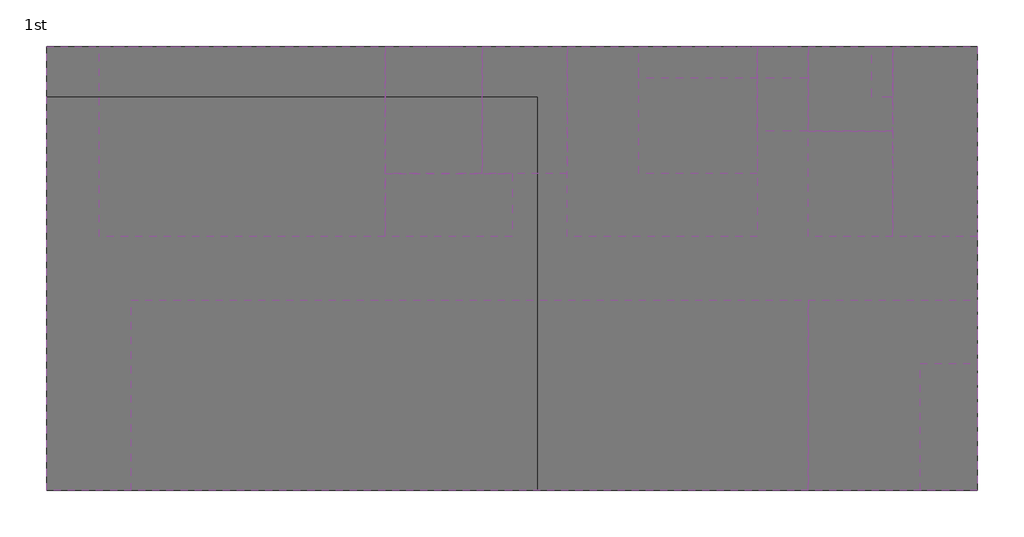
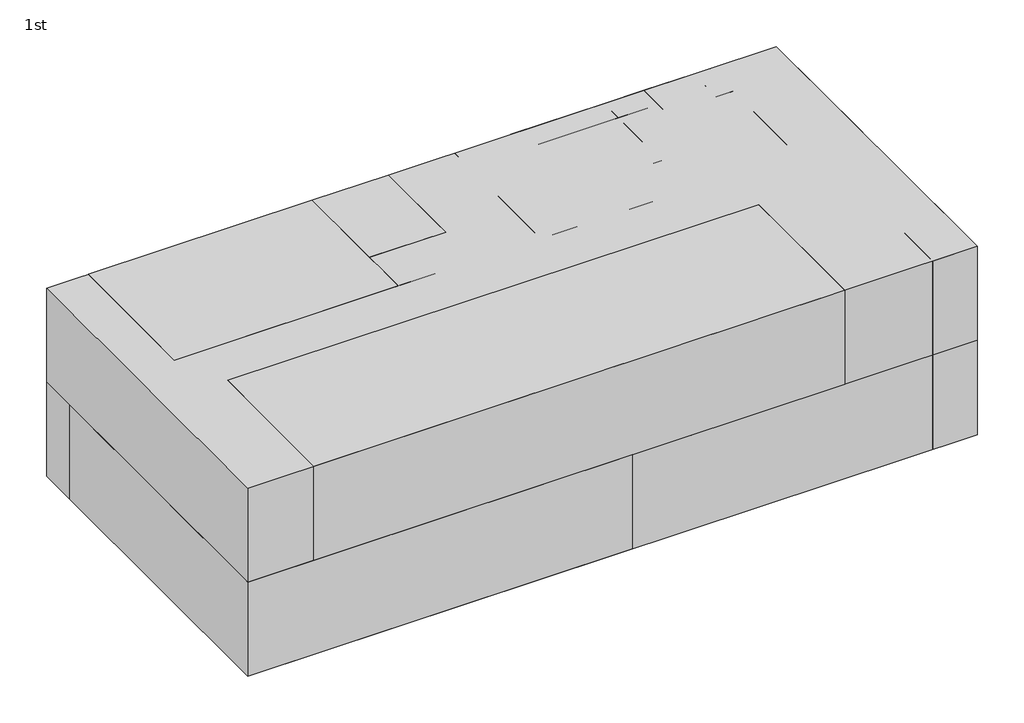
# One storey: 23 proxies.
"""IFC4 building model written with IfcOpenShell, lengths in millimetres."""

import ifcopenshell
import ifcopenshell.guid

model = None  # the IFC model being written
_history = None  # IfcOwnerHistory: only IFC2X3 demands one
_inside = {}  # id of a spatial element -> (the spatial element, [elements in it])
_under = {}  # id of a project, library or spatial element -> (it, [spatial elements below it])
_declared = {}  # id of a project -> (the project, [libraries it declares])
_typed = {}  # id of a type object -> (the type object, [elements of that type])
_made_of = {}  # id of a material, layer set ... -> (it, [elements and type objects made of it])


def new_model(schema):
    """Start an empty IFC model of exactly this schema.

    Asked for "IFC4X3", IfcOpenShell would pick the latest addendum, in which some entities
    have other attributes; the version numbers below select the first issue.
    IFC2X3 requires an IfcOwnerHistory on every rooted entity: one is made here for all.
    """
    global model, _history
    if schema == "IFC4X3":
        model = ifcopenshell.file(schema_version=(4, 3, 0, 0))
    else:
        model = ifcopenshell.file(schema=schema)
    _inside.clear()
    _under.clear()
    _declared.clear()
    _typed.clear()
    _made_of.clear()
    _history = None
    if model.schema == "IFC2X3":
        org = make("IfcOrganization", Name="unknown")
        user = make(
            "IfcPersonAndOrganization",
            ThePerson=make("IfcPerson", FamilyName="unknown"),
            TheOrganization=org,
        )
        app = make(
            "IfcApplication",
            ApplicationDeveloper=org,
            Version="unknown",
            ApplicationFullName="unknown",
            ApplicationIdentifier="unknown",
        )
        _history = make(
            "IfcOwnerHistory",
            OwningUser=user,
            OwningApplication=app,
            ChangeAction="ADDED",
            CreationDate=0,
        )
    return model


def make(cls, **values):
    """One entity of the class cls with the attributes given. An attribute that is None is left unset."""
    return model.create_entity(
        cls, **{name: value for name, value in values.items() if value is not None}
    )


def rooted(cls, **values):
    """An entity with a GlobalId (a new one), such as an element, a storey or a relation."""
    return make(cls, GlobalId=ifcopenshell.guid.new(), OwnerHistory=_history, **values)


def si_unit(unit_type, name, prefix=None):
    """IfcSIUnit, for example si_unit("LENGTHUNIT", "METRE", prefix="MILLI")."""
    return make("IfcSIUnit", UnitType=unit_type, Prefix=prefix, Name=name)


def assignment(units):
    """IfcUnitAssignment: the units of a project."""
    return None if units is None else make("IfcUnitAssignment", Units=units)


def point(xyz):
    """IfcCartesianPoint."""
    return None if xyz is None else make("IfcCartesianPoint", Coordinates=xyz)


def direction(xyz):
    """IfcDirection."""
    return None if xyz is None else make("IfcDirection", DirectionRatios=xyz)


def frame(location, z_axis=None, x_axis=None):
    """IfcAxis2Placement3D, a coordinate frame: its origin and axes. An axis left out is left unset."""
    return make(
        "IfcAxis2Placement3D",
        Location=point(location),
        Axis=direction(z_axis),
        RefDirection=direction(x_axis),
    )


def origin():
    """The frame at (0, 0, 0) with its axes left unset."""
    return frame((0.0, 0.0, 0.0))


def origin_with_axes():
    """The frame at (0, 0, 0) with the z axis (0, 0, 1) and the x axis (1, 0, 0) written out."""
    return frame((0.0, 0.0, 0.0), z_axis=(0.0, 0.0, 1.0), x_axis=(1.0, 0.0, 0.0))


def place(relative_to, where):
    """IfcLocalPlacement: puts the frame where relative to a parent placement (None: the world)."""
    return make(
        "IfcLocalPlacement", PlacementRelTo=relative_to, RelativePlacement=where
    )


def context(
    kind, dimensions, precision=None, world=None, true_north=None, identifier=None
):
    """IfcGeometricRepresentationContext, for example the 3D "Model" context."""
    return make(
        "IfcGeometricRepresentationContext",
        ContextIdentifier=identifier,
        ContextType=kind,
        CoordinateSpaceDimension=dimensions,
        Precision=precision,
        WorldCoordinateSystem=world,
        TrueNorth=true_north,
    )


def project(units=None, contexts=None):
    """IfcProject with its units and contexts."""
    return rooted(
        "IfcProject",
        Name="project",
        RepresentationContexts=contexts,
        UnitsInContext=assignment(units),
    )


def spatial(cls, under=None, at=None, **own):
    """A site, building, storey or space (cls), placed at a placement, below another one or the project."""
    s = rooted(cls, ObjectPlacement=at, **own)
    if under is not None:
        _under.setdefault(under.id(), (under, []))[1].append(s)
    return s


def polyline(points):
    """IfcPolyline through the points."""
    return make("IfcPolyline", Points=[point(p) for p in points])


def outline(outer, holes=None, kind="AREA"):
    """IfcArbitraryClosedProfileDef: a profile drawn as a closed curve; with holes, ...WithVoids."""
    if holes is None:
        return make("IfcArbitraryClosedProfileDef", ProfileType=kind, OuterCurve=outer)
    return make(
        "IfcArbitraryProfileDefWithVoids",
        ProfileType=kind,
        OuterCurve=outer,
        InnerCurves=holes,
    )


def extrude(swept, where, along, depth):
    """IfcExtrudedAreaSolid: the profile swept, set in the frame where, extruded along a direction by depth."""
    return make(
        "IfcExtrudedAreaSolid",
        SweptArea=swept,
        Position=where,
        ExtrudedDirection=direction(along),
        Depth=depth,
    )


def shape(context_of_items, identifier, shape_type, items):
    """IfcShapeRepresentation: the items that make up one representation, for example the "Body"."""
    return make(
        "IfcShapeRepresentation",
        ContextOfItems=context_of_items,
        RepresentationIdentifier=identifier,
        RepresentationType=shape_type,
        Items=items,
    )


def source(mapping_origin, context_of_items, identifier, shape_type, items):
    """IfcRepresentationMap: a shape defined once, which mapped items show again and again."""
    return make(
        "IfcRepresentationMap",
        MappingOrigin=mapping_origin,
        MappedRepresentation=shape(context_of_items, identifier, shape_type, items),
    )


def transform(
    local_origin,
    x_axis=None,
    y_axis=None,
    z_axis=None,
    scale=None,
    scale2=None,
    scale3=None,
    uniform=True,
):
    """IfcCartesianTransformationOperator3D, or its non-uniform kind. x_axis, y_axis, z_axis: its Axis1, 2, 3."""
    if uniform:
        return make(
            "IfcCartesianTransformationOperator3D",
            Axis1=direction(x_axis),
            Axis2=direction(y_axis),
            LocalOrigin=point(local_origin),
            Scale=scale,
            Axis3=direction(z_axis),
        )
    return make(
        "IfcCartesianTransformationOperator3DnonUniform",
        Axis1=direction(x_axis),
        Axis2=direction(y_axis),
        LocalOrigin=point(local_origin),
        Scale=scale,
        Axis3=direction(z_axis),
        Scale2=scale2,
        Scale3=scale3,
    )


def mapped(mapping_source, mapping_target):
    """IfcMappedItem: shows the shape of a source again, moved by a transform."""
    return make(
        "IfcMappedItem", MappingSource=mapping_source, MappingTarget=mapping_target
    )


def made_of(thing, what):
    """Note that an element or type object is made of a material, layer set ...; save() writes the relation."""
    if what is not None:
        _made_of.setdefault(what.id(), (what, []))[1].append(thing)
    return thing


def element(
    cls,
    number,
    at=None,
    inside=None,
    cuts=None,
    type_object=None,
    material=None,
    context=None,
    identifier="Body",
    shape_type=None,
    held_by="IfcProductDefinitionShape",
    body=None,
    shapes=None,
    **own,
):
    """One element of the class cls, such as IfcWall. Its Tag is "e" and its number.

    at: its placement. inside: the storey or other place that contains it. cuts: it is an
    opening in that element (IfcRelVoidsElement). A single representation is given by context,
    identifier, shape_type and body (its items); several are given by shapes. held_by: the class
    of the entity that holds the representations. save() writes the other relations.
    """
    e = rooted(cls, Tag="e%d" % number, ObjectPlacement=at, **own)
    if body is not None:
        shapes = [shape(context, identifier, shape_type, body)]
    if shapes is not None:
        e.Representation = make(held_by, Representations=shapes)
    if inside is not None:
        _inside.setdefault(inside.id(), (inside, []))[1].append(e)
    if cuts is not None:
        rooted(
            "IfcRelVoidsElement", RelatingBuildingElement=cuts, RelatedOpeningElement=e
        )
    if type_object is not None:
        _typed.setdefault(type_object.id(), (type_object, []))[1].append(e)
    return made_of(e, material)


def aggregate(whole, parts):
    """IfcRelAggregates: a whole, such as a stair, and the parts it consists of."""
    return rooted("IfcRelAggregates", RelatingObject=whole, RelatedObjects=parts)


def save(model, path):
    """Write the relations noted so far, then the file.

    IfcRelAggregates (storeys below a building ...), IfcRelContainedInSpatialStructure (elements
    in a storey), IfcRelDefinesByType, IfcRelAssociatesMaterial and IfcRelDeclares: one each for
    every whole, place, type object, material and project.
    """
    for whole, parts in _under.values():
        aggregate(whole, parts)
    for where, things in _inside.values():
        rooted(
            "IfcRelContainedInSpatialStructure",
            RelatedElements=things,
            RelatingStructure=where,
        )
    for kind, things in _typed.values():
        rooted("IfcRelDefinesByType", RelatedObjects=things, RelatingType=kind)
    for what, things in _made_of.values():
        rooted("IfcRelAssociatesMaterial", RelatedObjects=things, RelatingMaterial=what)
    for by, libraries in _declared.values():
        rooted("IfcRelDeclares", RelatingContext=by, RelatedDefinitions=libraries)
    model.write(path)


def generic_models_29bcd6f9(model_context):
    return source(origin(), model_context, "Body", "SweptSolid", [
        extrude(outline(polyline([(2000.0, 4500.0), (2000.0, -4500.0), (-2000.0, -4500.0), (-2000.0, 4500.0), (2000.0, 4500.0)])), origin_with_axes(), (0.0, 0.0, 1.0), 6000.0),
    ])


def generic_models_d82b1902(model_context):
    return source(origin(), model_context, "Body", "SweptSolid", [
        extrude(outline(polyline([(9300.0, 11600.0), (9300.0, -11600.0), (-9300.0, -11600.0), (-9300.0, 11600.0), (9300.0, 11600.0)])), origin_with_axes(), (0.0, 0.0, 1.0), 6000.0),
    ])


def generic_models_5634f436(model_context):
    return source(origin(), model_context, "Body", "SweptSolid", [
        extrude(outline(polyline([(1350.0, 3000.0), (1350.0, -3000.0), (-1350.0, -3000.0), (-1350.0, 3000.0), (1350.0, 3000.0)])), origin_with_axes(), (0.0, 0.0, 1.0), 6000.0),
    ])


def generic_models_57c7875f(model_context):
    return source(origin(), model_context, "Body", "SweptSolid", [
        extrude(outline(polyline([(4500.0, 16000.0), (4500.0, -16000.0), (-4500.0, -16000.0), (-4500.0, 16000.0), (4500.0, 16000.0)])), origin_with_axes(), (0.0, 0.0, 1.0), 6000.0),
    ])


def generic_models_7bff30ad(model_context):
    return source(origin(), model_context, "Body", "SweptSolid", [
        extrude(outline(polyline([(2000.0, 2000.0), (2000.0, -2000.0), (-2000.0, -2000.0), (-2000.0, 2000.0), (2000.0, 2000.0)])), origin_with_axes(), (0.0, 0.0, 1.0), 6000.0),
    ])


def generic_models_5b7b272c(model_context):
    return source(origin(), model_context, "Body", "SweptSolid", [
        extrude(outline(polyline([(2000.0, 2500.0), (2000.0, -2500.0), (-2000.0, -2500.0), (-2000.0, 2500.0), (2000.0, 2500.0)])), origin_with_axes(), (0.0, 0.0, 1.0), 6000.0),
    ])


def generic_models_47b98be1(model_context):
    return source(origin(), model_context, "Body", "SweptSolid", [
        extrude(outline(polyline([(1200.0, 2000.0), (1200.0, -2000.0), (-1200.0, -2000.0), (-1200.0, 2000.0), (1200.0, 2000.0)])), origin_with_axes(), (0.0, 0.0, 1.0), 6000.0),
    ])


def generic_models_7a053eeb(model_context):
    return source(origin(), model_context, "Body", "SweptSolid", [
        extrude(outline(polyline([(1200.0, 750.0), (1200.0, -750.0), (-1200.0, -750.0), (-1200.0, 750.0), (1200.0, 750.0)])), origin_with_axes(), (0.0, 0.0, 1.0), 6000.0),
    ])


def generic_models_ec17d728(model_context):
    return source(origin(), model_context, "Body", "SweptSolid", [
        extrude(outline(polyline([(2800.0, 3000.0), (2800.0, -3000.0), (-2800.0, -3000.0), (-2800.0, 3000.0), (2800.0, 3000.0)])), origin_with_axes(), (0.0, 0.0, 1.0), 6000.0),
    ])


def generic_models_85897e09(model_context):
    return source(origin(), model_context, "Body", "SweptSolid", [
        extrude(outline(polyline([(2800.0, 750.0), (2800.0, -750.0), (-2800.0, -750.0), (-2800.0, 750.0), (2800.0, 750.0)])), origin_with_axes(), (0.0, 0.0, 1.0), 6000.0),
    ])


def generic_models_b79df083(model_context):
    return source(origin(), model_context, "Body", "SweptSolid", [
        extrude(outline(polyline([(4500.0, 4500.0), (4500.0, -4500.0), (-4500.0, -4500.0), (-4500.0, 4500.0), (4500.0, 4500.0)])), origin_with_axes(), (0.0, 0.0, 1.0), 6000.0),
    ])


def generic_models_98b71764(model_context):
    return source(origin(), model_context, "Body", "SweptSolid", [
        extrude(outline(polyline([(2000.0, 3000.0), (2000.0, -3000.0), (-2000.0, -3000.0), (-2000.0, 3000.0), (2000.0, 3000.0)])), origin_with_axes(), (0.0, 0.0, 1.0), 6000.0),
    ])


def generic_models_1a87c0f4(model_context):
    return source(origin(), model_context, "Body", "SweptSolid", [
        extrude(outline(polyline([(2300.0, 3000.0), (2300.0, -3000.0), (-2300.0, -3000.0), (-2300.0, 3000.0), (2300.0, 3000.0)])), origin_with_axes(), (0.0, 0.0, 1.0), 6000.0),
    ])


def generic_models_df3bc381(model_context):
    return source(origin(), model_context, "Body", "SweptSolid", [
        extrude(outline(polyline([(4500.0, 6750.0), (4500.0, -6750.0), (-4500.0, -6750.0), (-4500.0, 6750.0), (4500.0, 6750.0)])), origin_with_axes(), (0.0, 0.0, 1.0), 6000.0),
    ])


def generic_models_542cc789(model_context):
    return source(origin(), model_context, "Body", "SweptSolid", [
        extrude(outline(polyline([(1500.0, 3000.0), (1500.0, -3000.0), (-1500.0, -3000.0), (-1500.0, 3000.0), (1500.0, 3000.0)])), origin_with_axes(), (0.0, 0.0, 1.0), 6000.0),
    ])


def generic_models_4d084078(model_context):
    return source(origin(), model_context, "Body", "SweptSolid", [
        extrude(outline(polyline([(4000.0, 4500.0), (4000.0, -4500.0), (-4000.0, -4500.0), (-4000.0, 4500.0), (4000.0, 4500.0)])), origin_with_axes(), (0.0, 0.0, 1.0), 6000.0),
    ])


def generic_models_7e8091d6(model_context):
    return source(origin(), model_context, "Body", "SweptSolid", [
        extrude(outline(polyline([(22000.0, 10500.0), (22000.0, -10500.0), (-22000.0, -10500.0), (-22000.0, 10500.0), (22000.0, 10500.0)])), origin_with_axes(), (0.0, 0.0, 1.0), 6000.0),
    ])


def generic_models_b146db3b(model_context):
    return source(origin(), model_context, "Body", "SweptSolid", [
        extrude(outline(polyline([(10500.0, 22000.0), (10500.0, -22000.0), (-10500.0, -22000.0), (-10500.0, 22000.0), (10500.0, 22000.0)])), origin_with_axes(), (0.0, 0.0, 1.0), 6000.0),
    ])


def generic_models_21888712(model_context):
    return source(origin(), model_context, "Body", "SweptSolid", [
        extrude(outline(polyline([(500.0, 1200.0), (500.0, -1200.0), (-500.0, -1200.0), (-500.0, 1200.0), (500.0, 1200.0)])), origin_with_axes(), (0.0, 0.0, 1.0), 6000.0),
    ])


model = new_model("IFC4")

# Units and contexts
model_context = context("Model", 3, world=origin())
ifc_project = project(units=[si_unit("LENGTHUNIT", "METRE", prefix="MILLI")], contexts=[model_context])

# Site, building, storey
site = spatial("IfcSite", under=ifc_project)
building = spatial("IfcBuilding", under=site)
storey = spatial("IfcBuildingStorey", under=building, Name="1st", Elevation=6000.0)

# Proxies
placement = place(None, origin())
element("IfcBuildingElementProxy", 1, Name="Space Planning Box_hec : Space Planning Box_hec", ObjectType="Space Planning Box_hec : Space Planning Box_hec", at=placement, inside=storey, context=model_context, shape_type="SweptSolid", body=[
    extrude(outline(polyline([(89459.6521483, 163923.8614395), (68659.6521483, 163923.8614395), (68659.6521483, 182523.8614395), (85459.6521483, 182523.8614395), (85459.6521483, 175923.8614395), (89459.6521483, 175923.8614395), (89459.6521483, 163923.8614395)])), frame((0.0, 0.0, 6000.0), z_axis=(0.0, 0.0, 1.0), x_axis=(1.0, 0.0, 0.0)), (0.0, 0.0, 1.0), 6000.0),
])
element("IfcBuildingElementProxy", 2, Name="Space Planning Box_hec : Space Planning Box_hec", ObjectType="Space Planning Box_hec : Space Planning Box_hec", at=placement, inside=storey, context=model_context, shape_type="SweptSolid", body=[
    extrude(outline(polyline([(89459.6521483, 184923.8614395), (89459.6521483, 175923.8614395), (85459.6521483, 175923.8614395), (85459.6521483, 184923.8614395), (89459.6521483, 184923.8614395)])), frame((0.0, 0.0, 6000.0), z_axis=(0.0, 0.0, 1.0), x_axis=(1.0, 0.0, 0.0)), (0.0, 0.0, 1.0), 6000.0),
])
generic_models_shape = generic_models_29bcd6f9(model_context)
element("IfcBuildingElementProxy", 3, Name="Space Planning Box_hec : Space Planning Box_hec", ObjectType="Space Planning Box_hec : Space Planning Box_hec", at=placement, inside=storey, context=model_context, shape_type="MappedRepresentation", body=[
    mapped(generic_models_shape, transform((87459.6521483, 180423.8614395, 12000.0), x_axis=(1.0, 0.0, 0.0), y_axis=(0.0, 1.0, 0.0), z_axis=(0.0, 0.0, 1.0))),
])
generic_models_2_shape = generic_models_d82b1902(model_context)
element("IfcBuildingElementProxy", 4, Name="Space Planning Box_hec : Space Planning Box_hec", ObjectType="Space Planning Box_hec : Space Planning Box_hec", at=placement, inside=storey, context=model_context, shape_type="MappedRepresentation", body=[
    mapped(generic_models_2_shape, transform((57059.6521483, 173223.8614395, 6000.0), x_axis=(0.0, -1.0, 0.0), y_axis=(1.0, 0.0, 0.0), z_axis=(0.0, 0.0, 1.0))),
])
generic_models_3_shape = generic_models_5634f436(model_context)
element("IfcBuildingElementProxy", 5, Name="Space Planning Box_hec : Space Planning Box_hec", ObjectType="Space Planning Box_hec : Space Planning Box_hec", at=placement, inside=storey, context=model_context, shape_type="MappedRepresentation", body=[
    mapped(generic_models_3_shape, transform((88109.6521483, 166923.8614395, 6000.0), x_axis=(1.0, 0.0, 0.0), y_axis=(0.0, 1.0, 0.0), z_axis=(0.0, 0.0, 1.0))),
])
element("IfcBuildingElementProxy", 6, Name="Space Planning Box_hec : Space Planning Box_hec", ObjectType="Space Planning Box_hec : Space Planning Box_hec", at=placement, inside=storey, context=model_context, shape_type="MappedRepresentation", body=[
    mapped(generic_models_3_shape, transform((88109.6521483, 166923.8614395, 12000.0), x_axis=(1.0, 0.0, 0.0), y_axis=(0.0, 1.0, 0.0), z_axis=(0.0, 0.0, 1.0))),
])
generic_models_4_shape = generic_models_57c7875f(model_context)
element("IfcBuildingElementProxy", 7, Name="Space Planning Box_hec : Space Planning Box_hec", ObjectType="Space Planning Box_hec : Space Planning Box_hec", at=placement, inside=storey, context=model_context, shape_type="MappedRepresentation", body=[
    mapped(generic_models_4_shape, transform((65459.6521483, 168423.8614395, 12000.0), x_axis=(0.0, -1.0, 0.0), y_axis=(1.0, 0.0, 0.0), z_axis=(0.0, 0.0, 1.0))),
])
generic_models_5_shape = generic_models_7bff30ad(model_context)
element("IfcBuildingElementProxy", 8, Name="Space Planning Box_hec : Space Planning Box_hec", ObjectType="Space Planning Box_hec : Space Planning Box_hec", at=placement, inside=storey, context=model_context, shape_type="MappedRepresentation", body=[
    mapped(generic_models_5_shape, transform((83459.6521483, 182923.8614395, 12000.0), x_axis=(1.0, 0.0, 0.0), y_axis=(0.0, 1.0, 0.0), z_axis=(0.0, 0.0, 1.0))),
])
generic_models_6_shape = generic_models_5b7b272c(model_context)
element("IfcBuildingElementProxy", 9, Name="Space Planning Box_hec : Space Planning Box_hec", ObjectType="Space Planning Box_hec : Space Planning Box_hec", at=placement, inside=storey, context=model_context, shape_type="MappedRepresentation", body=[
    mapped(generic_models_6_shape, transform((83459.6521483, 178423.8614395, 12000.0), x_axis=(1.0, 0.0, 0.0), y_axis=(0.0, 1.0, 0.0), z_axis=(0.0, 0.0, 1.0))),
])
generic_models_7_shape = generic_models_47b98be1(model_context)
element("IfcBuildingElementProxy", 10, Name="Space Planning Box_hec : Space Planning Box_hec", ObjectType="Space Planning Box_hec : Space Planning Box_hec", at=placement, inside=storey, context=model_context, shape_type="MappedRepresentation", body=[
    mapped(generic_models_7_shape, transform((80259.6521483, 182923.8614395, 12000.0), x_axis=(1.0, 0.0, 0.0), y_axis=(0.0, 1.0, 0.0), z_axis=(0.0, 0.0, 1.0))),
])
generic_models_8_shape = generic_models_7a053eeb(model_context)
element("IfcBuildingElementProxy", 11, Name="Space Planning Box_hec : Space Planning Box_hec", ObjectType="Space Planning Box_hec : Space Planning Box_hec", at=placement, inside=storey, context=model_context, shape_type="MappedRepresentation", body=[
    mapped(generic_models_8_shape, transform((80259.6521483, 184173.8614395, 12000.0), x_axis=(1.0, 0.0, 0.0), y_axis=(0.0, 1.0, 0.0), z_axis=(0.0, 0.0, 1.0))),
])
generic_models_9_shape = generic_models_ec17d728(model_context)
element("IfcBuildingElementProxy", 12, Name="Space Planning Box_hec : Space Planning Box_hec", ObjectType="Space Planning Box_hec : Space Planning Box_hec", at=placement, inside=storey, context=model_context, shape_type="MappedRepresentation", body=[
    mapped(generic_models_9_shape, transform((76259.6521483, 181923.8614395, 12000.0), x_axis=(1.0, 0.0, 0.0), y_axis=(0.0, 1.0, 0.0), z_axis=(0.0, 0.0, 1.0))),
])
generic_models_10_shape = generic_models_85897e09(model_context)
element("IfcBuildingElementProxy", 13, Name="Space Planning Box_hec : Space Planning Box_hec", ObjectType="Space Planning Box_hec : Space Planning Box_hec", at=placement, inside=storey, context=model_context, shape_type="MappedRepresentation", body=[
    mapped(generic_models_10_shape, transform((76259.6521483, 184173.8614395, 12000.0), x_axis=(1.0, 0.0, 0.0), y_axis=(0.0, 1.0, 0.0), z_axis=(0.0, 0.0, 1.0))),
])
generic_models_11_shape = generic_models_b79df083(model_context)
element("IfcBuildingElementProxy", 14, Name="Space Planning Box_hec : Space Planning Box_hec", ObjectType="Space Planning Box_hec : Space Planning Box_hec", at=placement, inside=storey, context=model_context, shape_type="MappedRepresentation", body=[
    mapped(generic_models_11_shape, transform((74559.6521483, 180423.8614395, 12000.0), x_axis=(1.0, 0.0, 0.0), y_axis=(0.0, 1.0, 0.0), z_axis=(0.0, 0.0, 1.0))),
])
generic_models_12_shape = generic_models_98b71764(model_context)
element("IfcBuildingElementProxy", 15, Name="Space Planning Box_hec : Space Planning Box_hec", ObjectType="Space Planning Box_hec : Space Planning Box_hec", at=placement, inside=storey, context=model_context, shape_type="MappedRepresentation", body=[
    mapped(generic_models_12_shape, transform((68059.6521483, 181923.8614395, 12000.0), x_axis=(1.0, 0.0, 0.0), y_axis=(0.0, 1.0, 0.0), z_axis=(0.0, 0.0, 1.0))),
])
generic_models_13_shape = generic_models_1a87c0f4(model_context)
element("IfcBuildingElementProxy", 16, Name="Space Planning Box_hec : Space Planning Box_hec", ObjectType="Space Planning Box_hec : Space Planning Box_hec", at=placement, inside=storey, context=model_context, shape_type="MappedRepresentation", body=[
    mapped(generic_models_13_shape, transform((63759.6521483, 181923.8614395, 12000.0), x_axis=(1.0, 0.0, 0.0), y_axis=(0.0, 1.0, 0.0), z_axis=(0.0, 0.0, 1.0))),
])
generic_models_14_shape = generic_models_df3bc381(model_context)
element("IfcBuildingElementProxy", 17, Name="Space Planning Box_hec : Space Planning Box_hec", ObjectType="Space Planning Box_hec : Space Planning Box_hec", at=placement, inside=storey, context=model_context, shape_type="MappedRepresentation", body=[
    mapped(generic_models_14_shape, transform((54709.6521483, 180423.8614395, 12000.0), x_axis=(0.0, -1.0, 0.0), y_axis=(1.0, 0.0, 0.0), z_axis=(0.0, 0.0, 1.0))),
])
generic_models_15_shape = generic_models_542cc789(model_context)
element("IfcBuildingElementProxy", 18, Name="Space Planning Box_hec : Space Planning Box_hec", ObjectType="Space Planning Box_hec : Space Planning Box_hec", at=placement, inside=storey, context=model_context, shape_type="MappedRepresentation", body=[
    mapped(generic_models_15_shape, transform((64459.6521483, 177423.8614395, 12000.0), x_axis=(0.0, -1.0, 0.0), y_axis=(1.0, 0.0, 0.0), z_axis=(0.0, 0.0, 1.0))),
])
generic_models_16_shape = generic_models_4d084078(model_context)
element("IfcBuildingElementProxy", 19, Name="Space Planning Box_hec : Space Planning Box_hec", ObjectType="Space Planning Box_hec : Space Planning Box_hec", at=placement, inside=storey, context=model_context, shape_type="MappedRepresentation", body=[
    mapped(generic_models_16_shape, transform((85459.6521483, 168423.8614395, 12000.0), x_axis=(1.0, 0.0, 0.0), y_axis=(0.0, 1.0, 0.0), z_axis=(0.0, 0.0, 1.0))),
])
generic_models_17_shape = generic_models_7e8091d6(model_context)
element("IfcBuildingElementProxy", 20, Name="Space Planning Box_hec : Space Planning Box_hec", ObjectType="Space Planning Box_hec : Space Planning Box_hec", at=placement, inside=storey, context=model_context, shape_type="MappedRepresentation", body=[
    mapped(generic_models_17_shape, transform((67459.6521483, 174423.8614395, 12000.0), x_axis=(1.0, 0.0, 0.0), y_axis=(0.0, 1.0, 0.0), z_axis=(0.0, 0.0, 1.0))),
])
generic_models_18_shape = generic_models_b146db3b(model_context)
element("IfcBuildingElementProxy", 21, Name="Space Planning Box_hec : Space Planning Box_hec", ObjectType="Space Planning Box_hec : Space Planning Box_hec", at=placement, inside=storey, context=model_context, shape_type="MappedRepresentation", body=[
    mapped(generic_models_18_shape, transform((67459.6521483, 174423.8614395, 6000.0), x_axis=(0.0, -1.0, 0.0), y_axis=(1.0, 0.0, 0.0), z_axis=(0.0, 0.0, 1.0))),
])
generic_models_19_shape = generic_models_21888712(model_context)
element("IfcBuildingElementProxy", 22, Name="Space Planning Box_hec : Space Planning Box_hec", ObjectType="Space Planning Box_hec : Space Planning Box_hec", at=placement, inside=storey, context=model_context, shape_type="MappedRepresentation", body=[
    mapped(generic_models_19_shape, transform((84959.6521483, 183723.8614395, 6000.0), x_axis=(1.0, 0.0, 0.0), y_axis=(0.0, 1.0, 0.0), z_axis=(0.0, 0.0, 1.0))),
])
element("IfcBuildingElementProxy", 23, Name="Space Planning Box_hec : Space Planning Box_hec", ObjectType="Space Planning Box_hec : Space Planning Box_hec", at=placement, inside=storey, context=model_context, shape_type="MappedRepresentation", body=[
    mapped(generic_models_19_shape, transform((84959.6521483, 183723.8614395, 12000.0), x_axis=(1.0, 0.0, 0.0), y_axis=(0.0, 1.0, 0.0), z_axis=(0.0, 0.0, 1.0))),
])

save(model, "model.ifc")

# Revit data of these elements
# Type "Space Planning Box_hec : Space Planning Box_hec"
#   Type Comments = "..."
#   Room Name [instance default] = "?"
#   Interior Finish [instance default] = ""
#   Exterior Finish [instance default] = ""
#   Department [instance default] = ""
#   Assembly Code = "..."
#   Width [instance default] = 1524 mm
#   Program Area [instance default] = 0.00 m²
#   Length [instance default] = 1524 mm
#   Height [instance default] = 1524 mm
#   Area [instance default] = 2.32258 m²
#   Fill Color [instance default] = Cyan
#   Default Elevation = 0
# Element 1 (IfcBuildingElementProxy, "Space Planning Box_hec : Space Planning Box_hec")
#   Room Name = "Electrical Room"
#   Interior Finish = "IF1"
#   Exterior Finish = "EF1"
#   Department = "EL"
#   Width = 18600 mm
#   Program Area = 238.08 m²
#   Length = 20800 mm
#   Height = 6000 mm
#   Area = 386.88 m²
#   Fill Color = Blue
#   Phase Created = New Construction
#   Materials on its faces: "Blue"
# Element 2 (IfcBuildingElementProxy, "Space Planning Box_hec : Space Planning Box_hec")
#   Room Name = "Stairway"
#   Interior Finish = "IF2"
#   Exterior Finish = "EF1"
#   Department = "AR"
#   Width = 4000 mm
#   Program Area = 36.00 m²
#   Length = 9000 mm
#   Height = 6000 mm
#   Area = 36.00 m²
#   Fill Color = Lavender
#   Phase Created = New Construction
#   Materials on its faces: "Lavender"
# Element 3 (IfcBuildingElementProxy, "Space Planning Box_hec : Space Planning Box_hec")
#   Room Name = "Stairway"
#   Interior Finish = "IF2"
#   Exterior Finish = "EF1"
#   Department = "AR"
#   Width = 4000 mm
#   Program Area = 38.00 m²
#   Length = 9000 mm
#   Height = 6000 mm
#   Area = 36.00 m²
#   Fill Color = Lavender
#   Phase Created = New Construction
#   Materials on its faces: "Lavender"
# Element 4 (IfcBuildingElementProxy, "Space Planning Box_hec : Space Planning Box_hec")
#   Room Name = "Electronic Room"
#   Interior Finish = "IF1"
#   Exterior Finish = "EF1"
#   Department = "CI"
#   Width = 18600 mm
#   Program Area = 431.52 m²
#   Length = 23200 mm
#   Height = 6000 mm
#   Area = 431.52 m²
#   Fill Color = Lime
#   Phase Created = New Construction
#   Materials on its faces: "Lime"
# Elements 5, 6 (IfcBuildingElementProxy, "Space Planning Box_hec : Space Planning Box_hec")
#   Room Name = "Duct Shaft"
#   Interior Finish = "NA"
#   Exterior Finish = "EF1"
#   Department = "HV"
#   Width = 2700 mm
#   Program Area = 16.20 m²
#   Length = 6000 mm
#   Height = 6000 mm
#   Area = 16.20 m²
#   Fill Color = Pink
#   Phase Created = New Construction
#   Materials on its faces: "Pink"
# Element 7 (IfcBuildingElementProxy, "Space Planning Box_hec : Space Planning Box_hec")
#   Room Name = "Central Control Room"
#   Interior Finish = "IF3"
#   Exterior Finish = "EF1"
#   Department = "CI"
#   Width = 9000 mm
#   Program Area = 288.00 m²
#   Length = 32000 mm
#   Height = 6000 mm
#   Area = 288.00 m²
#   Fill Color = Lime
#   Phase Created = New Construction
#   Materials on its faces: "Lime"
# Element 8 (IfcBuildingElementProxy, "Space Planning Box_hec : Space Planning Box_hec")
#   Room Name = "Toilet (F)"
#   Interior Finish = "IF5"
#   Exterior Finish = "EF1"
#   Department = "AR"
#   Width = 4000 mm
#   Program Area = 72.00 m²
#   Length = 4000 mm
#   Height = 6000 mm
#   Area = 16.00 m²
#   Fill Color = Lavender
#   Phase Created = New Construction
#   Materials on its faces: "Lavender"
# Element 9 (IfcBuildingElementProxy, "Space Planning Box_hec : Space Planning Box_hec")
#   Room Name = "Toilet (M)"
#   Interior Finish = "IF5"
#   Exterior Finish = "EF1"
#   Department = "AR"
#   Width = 4000 mm
#   Program Area = 72.00 m²
#   Length = 5000 mm
#   Height = 6000 mm
#   Area = 20.00 m²
#   Fill Color = Lavender
#   Phase Created = New Construction
#   Materials on its faces: "Lavender"
# Element 10 (IfcBuildingElementProxy, "Space Planning Box_hec : Space Planning Box_hec")
#   Room Name = "Locker Room (F)"
#   Interior Finish = "IF2-1"
#   Exterior Finish = "EF1"
#   Department = "AR"
#   Width = 2400 mm
#   Program Area = 31.50 m²
#   Length = 4000 mm
#   Height = 6000 mm
#   Area = 9.60 m²
#   Fill Color = Lavender
#   Phase Created = New Construction
#   Materials on its faces: "Lavender"
# Element 11 (IfcBuildingElementProxy, "Space Planning Box_hec : Space Planning Box_hec")
#   Room Name = "Shower Room (F)"
#   Interior Finish = "IF5"
#   Exterior Finish = "EF1"
#   Department = "AR"
#   Width = 2400 mm
#   Program Area = 31.50 m²
#   Length = 1500 mm
#   Height = 6000 mm
#   Area = 3.60 m²
#   Fill Color = Lavender
#   Phase Created = New Construction
#   Materials on its faces: "Lavender"
# Element 12 (IfcBuildingElementProxy, "Space Planning Box_hec : Space Planning Box_hec")
#   Room Name = "Locker Room (M)"
#   Interior Finish = "IF2-1"
#   Exterior Finish = "EF1"
#   Department = "AR"
#   Width = 5600 mm
#   Program Area = 31.50 m²
#   Length = 6000 mm
#   Height = 6000 mm
#   Area = 33.60 m²
#   Fill Color = Lavender
#   Phase Created = New Construction
#   Materials on its faces: "Lavender"
# Element 13 (IfcBuildingElementProxy, "Space Planning Box_hec : Space Planning Box_hec")
#   Room Name = "Shower Room (M)"
#   Interior Finish = "IF5"
#   Exterior Finish = "EF1"
#   Department = "AR"
#   Width = 5600 mm
#   Program Area = 31.50 m²
#   Length = 1500 mm
#   Height = 6000 mm
#   Area = 8.40 m²
#   Fill Color = Lavender
#   Phase Created = New Construction
#   Materials on its faces: "Lavender"
# Element 14 (IfcBuildingElementProxy, "Space Planning Box_hec : Space Planning Box_hec")
#   Room Name = "Kitch & Lunch Room"
#   Interior Finish = "IF2-1"
#   Exterior Finish = "EF1"
#   Department = "AR"
#   Width = 9000 mm
#   Program Area = 31.50 m²
#   Length = 9000 mm
#   Height = 6000 mm
#   Area = 81.00 m²
#   Fill Color = Lavender
#   Phase Created = New Construction
#   Materials on its faces: "Lavender"
# Element 15 (IfcBuildingElementProxy, "Space Planning Box_hec : Space Planning Box_hec")
#   Room Name = "Shift Office Room"
#   Interior Finish = "IF2-1"
#   Exterior Finish = "EF1"
#   Department = "AR"
#   Width = 4000 mm
#   Program Area = 43.20 m²
#   Length = 6000 mm
#   Height = 6000 mm
#   Area = 24.00 m²
#   Fill Color = Lavender
#   Phase Created = New Construction
#   Materials on its faces: "Lavender"
# Element 16 (IfcBuildingElementProxy, "Space Planning Box_hec : Space Planning Box_hec")
#   Room Name = "Document Room"
#   Interior Finish = "IF2-1"
#   Exterior Finish = "EF1"
#   Department = "AR"
#   Width = 4600 mm
#   Program Area = 48.00 m²
#   Length = 6000 mm
#   Height = 6000 mm
#   Area = 27.60 m²
#   Fill Color = Lavender
#   Phase Created = New Construction
#   Materials on its faces: "Lavender"
# Element 17 (IfcBuildingElementProxy, "Space Planning Box_hec : Space Planning Box_hec")
#   Room Name = "Engineer Room"
#   Interior Finish = "IF3"
#   Exterior Finish = "EF1"
#   Department = "CI"
#   Width = 9000 mm
#   Program Area = 120.00 m²
#   Length = 13500 mm
#   Height = 6000 mm
#   Area = 121.50 m²
#   Fill Color = Lime
#   Phase Created = New Construction
#   Materials on its faces: "Lime"
# Element 18 (IfcBuildingElementProxy, "Space Planning Box_hec : Space Planning Box_hec")
#   Room Name = "LOTO Office Room"
#   Interior Finish = "IF2-1"
#   Exterior Finish = "EF1"
#   Department = "AR"
#   Width = 3000 mm
#   Program Area = 31.50 m²
#   Length = 6000 mm
#   Height = 6000 mm
#   Area = 18.00 m²
#   Fill Color = Lavender
#   Phase Created = New Construction
#   Materials on its faces: "Lavender"
# Element 19 (IfcBuildingElementProxy, "Space Planning Box_hec : Space Planning Box_hec")
#   Room Name = "Fire Gas Room"
#   Interior Finish = "IF1"
#   Exterior Finish = "EF1"
#   Department = "SF"
#   Width = 8000 mm
#   Program Area = 0.00 m²
#   Length = 9000 mm
#   Height = 6000 mm
#   Area = 72.00 m²
#   Fill Color = Cyan
#   Phase Created = New Construction
#   Materials on its faces: "Cyan"
# Element 20 (IfcBuildingElementProxy, "Space Planning Box_hec : Space Planning Box_hec")
#   Room Name = "Corridor"
#   Interior Finish = "IF2-1"
#   Exterior Finish = "EF1"
#   Department = "AR"
#   Width = 44000 mm
#   Program Area = 0.00 m²
#   Length = 21000 mm
#   Height = 6000 mm
#   Area = 924.00 m²
#   Fill Color = Lavender
#   Phase Created = New Construction
#   Materials on its faces: "Lavender"
# Element 21 (IfcBuildingElementProxy, "Space Planning Box_hec : Space Planning Box_hec")
#   Room Name = "Corridor"
#   Interior Finish = "IF2-1"
#   Exterior Finish = "EF1"
#   Department = "AR"
#   Width = 21000 mm
#   Program Area = 86.40 m²
#   Length = 44000 mm
#   Height = 6000 mm
#   Area = 924.00 m²
#   Fill Color = Lavender
#   Phase Created = New Construction
#   Materials on its faces: "Lavender"
# Elements 22, 23 (IfcBuildingElementProxy, "Space Planning Box_hec : Space Planning Box_hec")
#   Room Name = "Pipe Shaft"
#   Interior Finish = "NA"
#   Exterior Finish = "EF1"
#   Department = "HV"
#   Width = 1000 mm
#   Program Area = 2.50 m²
#   Length = 2400 mm
#   Height = 6000 mm
#   Area = 2.40 m²
#   Fill Color = Pink
#   Phase Created = New Construction
#   Materials on its faces: "Pink"
# Materials
#   "Cyan": class "Generic", colour RGB 0 255 255, transparency 0.2, Cost = 0
#   "Blue": class "Generic", colour RGB 0 0 255, transparency 0.2, Cost = 0
#   "Lavender": class "Generic", colour RGB 186 85 211, transparency 0.2, Cost = 0
#   "Lime": class "Generic", colour RGB 0 255 0, transparency 0.2, Cost = 0
#   "Pink": class "Generic", colour RGB 255 105 180, transparency 0.2, Cost = 0
